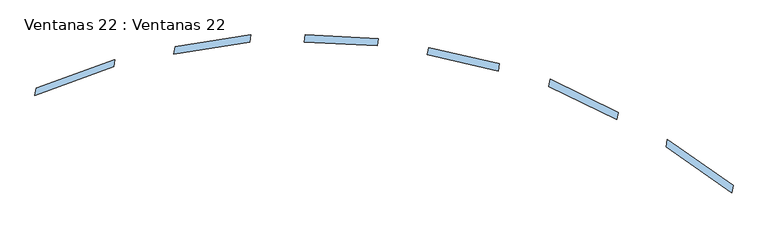
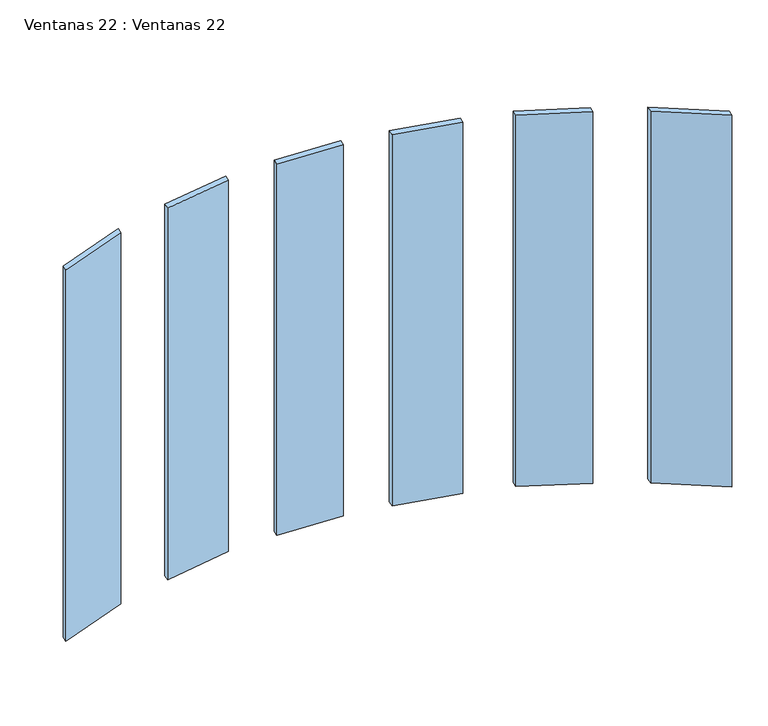
"""IFC4 building model written with IfcOpenShell, lengths in millimetres: window geometry, Ventanas 22 : Ventanas 22."""

from ifc_helpers import new_model, si_unit, frame, origin, place, context, project, spatial, polyline, outline, extrude, source, transform, mapped, element, save


def ventanas_22_ventanas_22_fe4727b4(model_context):
    return source(origin(), model_context, "Body", "SweptSolid", [
        extrude(outline(polyline([(5522.6851845, 8942.9284603), (5519.2122209, 8923.2323053), (5317.9864073, 8933.7781033), (5321.4593708, 8953.4742584), (5522.6851845, 8942.9284603)])), frame((0.0, 0.0, 6205.0301527), z_axis=(0.0, 0.0, 1.0), x_axis=(1.0, 0.0, 0.0)), (0.0, 0.0, 1.0), 1224.4032382),
        extrude(outline(polyline([(5855.6997174, 8873.5657625), (5852.2267539, 8853.8696074), (5657.0853063, 8898.9215604), (5660.5582699, 8918.6177155), (5855.6997174, 8873.5657625)])), frame((0.0, 0.0, 6205.0301527), z_axis=(0.0, 0.0, 1.0), x_axis=(1.0, 0.0, 0.0)), (0.0, 0.0, 1.0), 1224.4032382),
        extrude(outline(polyline([(6182.6278016, 8739.5789161), (6179.1548381, 8719.882761), (5992.1518502, 8811.0902123), (5995.6248137, 8830.7863674), (6182.6278016, 8739.5789161)])), frame((0.0, 0.0, 6205.0301527), z_axis=(0.0, 0.0, 1.0), x_axis=(1.0, 0.0, 0.0)), (0.0, 0.0, 1.0), 1224.4032382),
        extrude(outline(polyline([(4962.2216769, 8920.3845933), (5171.1416001, 8953.4742584), (5167.6686365, 8933.7781033), (4958.7487134, 8900.6884382), (4962.2216769, 8920.3845933)])), frame((0.0, 0.0, 6205.0301527), z_axis=(0.0, 0.0, 1.0), x_axis=(1.0, 0.0, 0.0)), (0.0, 0.0, 1.0), 1224.4032382),
        extrude(outline(polyline([(4579.4915042, 8806.1740915), (4796.5042193, 8885.1602603), (4793.0312557, 8865.4641052), (4576.0185407, 8786.4779365), (4579.4915042, 8806.1740915)])), frame((0.0, 0.0, 6205.0301527), z_axis=(0.0, 0.0, 1.0), x_axis=(1.0, 0.0, 0.0)), (0.0, 0.0, 1.0), 1224.4032382),
        extrude(outline(polyline([(6499.7009833, 8537.4487708), (6496.2280197, 8517.7526158), (6315.4611641, 8644.3269307), (6318.9341277, 8664.0230858), (6499.7009833, 8537.4487708)])), frame((0.0, 0.0, 6205.0301527), z_axis=(0.0, 0.0, 1.0), x_axis=(1.0, 0.0, 0.0)), (0.0, 0.0, 1.0), 1224.4032382),
    ])


if __name__ == "__main__":
    model = new_model("IFC4")
    model_context = context("Model", 3, world=origin())
    ifc_project = project(units=[si_unit("LENGTHUNIT", "METRE", prefix="MILLI")], contexts=[model_context])
    site = spatial("IfcSite", under=ifc_project)
    building = spatial("IfcBuilding", under=site)
    placement = place(None, origin())
    ventanas_22_ventanas_22_shape = ventanas_22_ventanas_22_fe4727b4(model_context)
    element("IfcWindow", 1, ObjectType="Ventanas 22 : Ventanas 22", at=placement, inside=building, context=model_context, shape_type="MappedRepresentation", body=[
        mapped(ventanas_22_ventanas_22_shape, transform((0.0, 0.0, 0.0), x_axis=(1.0, 0.0, 0.0), y_axis=(0.0, 1.0, 0.0), z_axis=(0.0, 0.0, 1.0))),
    ])
    save(model, "model.ifc")

# Revit data of these elements
# Type "Ventanas 22 : Ventanas 22"
#   Type Mark = "48"
# Element 1 (IfcWindow, "Ventanas 22 : Ventanas 22")
#   Materials on its faces: "VIDRIO"
# Materials
#   "VIDRIO": class "Genérico", colour RGB 120 120 120, transparency 0, Cost = 0
